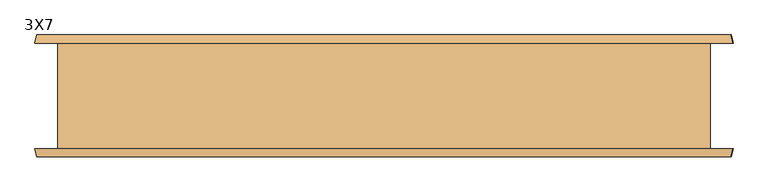
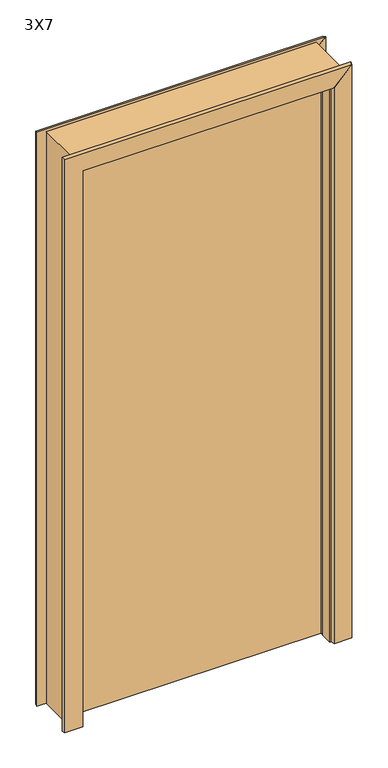
"""IFC4 building model written with IfcOpenShell, lengths in millimetres: door geometry, ASSA ABLOY BE_Doorset_Double Action Door_HardwareSet Info : 3X7."""

from ifc_helpers import new_model, si_unit, point, frame, frame_2d, origin, place, context, project, spatial, polyline, circle_curve, ellipse_curve, trimmed, segment, composite_curve, outline, extrude, faceted_brep, source, transform, mapped, element, save
from ifc_brep_helpers import plane_surface, revolved_surface, advanced_brep


def door_3x7_5d484fb7(model_context):
    return source(origin(), model_context, "Body", "SolidModel", [
        extrude(outline(composite_curve([segment(trimmed(circle_curve(frame_2d((376.3004472, 0.0)), 60.0), [point((430.8440078, 25.0))], [point((430.8440078, -25.0))], False, "CARTESIAN"), True, "CONTINUOUS"), segment(polyline([(430.8440078, -25.0), (-429.2, -25.0), (-429.2, 25.0), (430.8440078, 25.0)]), True, "CONTINUOUS")], self_intersect=False)), frame((0.0, 0.0, 4.0), z_axis=(0.0, 0.0, 1.0), x_axis=(1.0, 0.0, 0.0)), (0.0, 0.0, 1.0), 2096.0),
        advanced_brep(
        [(432.1999993, 29.0558097, 0.0), (432.1999993, 76.2, 0.0), (437.2, 76.2, 0.0), (440.2, 88.2, 0.0), (502.2, 88.2, 0.0), (505.2, 76.2, 0.0), (457.2, 76.2, 0.0), (457.2, -76.2, 0.0), (505.2, -76.2, 0.0), (502.2, -88.2, 0.0), (440.2, -88.2, 0.0), (437.2, -76.2, 0.0), (432.2, -76.2, 0.0), (432.2, -29.0558084, 0.0), (432.1999993, 29.0558097, 2049.9999993), (432.1999993, 76.2, 2049.9999993), (437.2, 76.2, 2055.0), (440.2, 88.2, 2058.0), (502.2, 88.2, 2120.0), (505.2, 76.2, 2123.0), (457.2, 76.2, 2075.0), (457.2, -76.2, 2075.0), (505.2, -76.2, 2123.0), (502.2, -88.2, 2120.0), (440.2, -88.2, 2058.0), (437.2, -76.2, 2055.0), (432.2, -76.2, 2050.0), (432.2, -29.0558084, 2050.0)],
        [
            (0, 1),
            (1, 2),
            (2, 3),
            (3, 4),
            (4, 5),
            (5, 6),
            (6, 7),
            (7, 8),
            (8, 9),
            (9, 10),
            (10, 11),
            (11, 12),
            (12, 13),
            (13, 0, circle_curve(frame((376.3004472, 0.0, 0.0), z_axis=(0.0, 0.0, 1.0), x_axis=(-1.0, 0.0, 0.0)), 63.0)),
            (0, 14),
            (14, 15),
            (15, 1),
            (15, 16),
            (16, 2),
            (16, 17),
            (17, 3),
            (17, 18),
            (18, 4),
            (18, 19),
            (19, 5),
            (19, 20),
            (20, 6),
            (20, 21),
            (21, 7),
            (21, 22),
            (22, 8),
            (22, 23),
            (23, 9),
            (23, 24),
            (24, 10),
            (24, 25),
            (25, 11),
            (25, 26),
            (26, 12),
            (26, 27),
            (27, 13),
            (27, 14, ellipse_curve(frame((376.3004472, 0.0, 1994.1004472), z_axis=(-0.7071067811865507, 0.0, 0.7071067811865445), x_axis=(0.7071067811865445, 0.0, 0.7071067811865505)), 89.0954544, 63.0)),
        ],
        [
            plane_surface(frame((457.2, 76.2, 0.0), z_axis=(0.0, 0.0, -1.0), x_axis=(0.0, -1.0, 0.0))),
            plane_surface(frame((432.1999993, 29.0558097, 0.0), z_axis=(-1.0, 0.0, 0.0), x_axis=(0.0, 0.0, 1.0))),
            plane_surface(frame((432.1999993, 76.2, 0.0), z_axis=(0.0, 1.0, 0.0), x_axis=(0.0, 0.0, 1.0))),
            plane_surface(frame((437.2, 76.2, 0.0), z_axis=(-0.9701425001453396, 0.24253562503630208, 0.0), x_axis=(0.0, 0.0, 1.0))),
            plane_surface(frame((440.2, 88.2, 0.0), z_axis=(0.0, 1.0, 0.0), x_axis=(0.0, 0.0, 1.0))),
            plane_surface(frame((502.2, 88.2, 0.0), z_axis=(0.9701425001453319, 0.24253562503633297, 0.0), x_axis=(0.0, 0.0, 1.0))),
            plane_surface(frame((505.2, 76.2, 0.0), z_axis=(0.0, -1.0, 0.0), x_axis=(0.0, 0.0, 1.0))),
            plane_surface(frame((457.2, 76.2, 0.0), z_axis=(1.0, 0.0, 0.0), x_axis=(0.0, 0.0, 1.0))),
            plane_surface(frame((457.2, -76.2, 0.0), z_axis=(0.0, 1.0, 0.0), x_axis=(0.0, 0.0, 1.0))),
            plane_surface(frame((505.2, -76.2, 0.0), z_axis=(0.9701425001453553, -0.24253562503623965, 0.0), x_axis=(0.0, 0.0, 1.0))),
            plane_surface(frame((502.2, -88.2, 0.0), z_axis=(0.0, -1.0, 0.0), x_axis=(0.0, 0.0, 1.0))),
            plane_surface(frame((440.2, -88.2, 0.0), z_axis=(-0.970142500145363, -0.24253562503620874, 0.0), x_axis=(0.0, 0.0, 1.0))),
            plane_surface(frame((437.2, -76.2, 0.0), z_axis=(0.0, -1.0, 0.0), x_axis=(0.0, 0.0, 1.0))),
            plane_surface(frame((432.2, -76.2, 0.0), z_axis=(-1.0, 0.0, 0.0), x_axis=(0.0, 0.0, 1.0))),
            revolved_surface(polyline([(313.3004472, 0.0, 2057.100447179137), (313.3004472, 0.0, 0.0)]), (376.3004472, 0.0, 0.0), (0.0, 0.0, 1.0)),
            plane_surface(frame((345.6190436, -88.2, 1963.4190436), z_axis=(-0.7071067811865507, 0.0, 0.7071067811865445), x_axis=(0.0, 1.0, 0.0))),
        ],
        [
            (0, [[1, 2, 3, 4, 5, 6, 7, 8, 9, 10, 11, 12, 13, 14]]),
            (1, [[-1, 15, 16, 17]]),
            (2, [[-2, -17, 18, 19]]),
            (3, [[-3, -19, 20, 21]]),
            (4, [[-4, -21, 22, 23]]),
            (5, [[-5, -23, 24, 25]]),
            (6, [[-6, -25, 26, 27]]),
            (7, [[-7, -27, 28, 29]]),
            (8, [[-8, -29, 30, 31]]),
            (9, [[-9, -31, 32, 33]]),
            (10, [[-10, -33, 34, 35]]),
            (11, [[-11, -35, 36, 37]]),
            (12, [[-12, -37, 38, 39]]),
            (13, [[-13, -39, 40, 41]]),
            (14, [[-14, -41, 42, -15]]),
            (15, [[-16, -42, -40, -38, -36, -34, -32, -30, -28, -26, -24, -22, -20, -18]]),
        ],
    ),
        faceted_brep([(-432.1999993, -76.2, 0.0), (-437.2, -76.2, 0.0), (-440.2, -88.2, 0.0), (-502.2, -88.2, 0.0), (-505.2, -76.2, 0.0), (-457.2, -76.2, 0.0), (-457.2, 76.2, 0.0), (-505.2, 76.2, 0.0), (-502.2, 88.2, 0.0), (-440.2, 88.2, 0.0), (-437.2, 76.2, 0.0), (-432.1999993, 76.2, 0.0), (-432.1999993, -76.2, 2049.9999993), (432.1999993, -76.2, 2049.9999993), (437.2, -76.2, 2055.0), (-437.2, -76.2, 2055.0), (-440.2, -88.2, 2058.0), (440.2, -88.2, 2058.0), (502.2, -88.2, 2120.0), (-502.2, -88.2, 2120.0), (-505.2, -76.2, 2123.0), (505.2, -76.2, 2123.0), (457.2, -76.2, 2075.0), (-457.2, -76.2, 2075.0), (-457.2, 76.2, 2075.0), (457.2, 76.2, 2075.0), (505.2, 76.2, 2123.0), (-505.2, 76.2, 2123.0), (-502.2, 88.2, 2120.0), (502.2, 88.2, 2120.0), (440.2, 88.2, 2058.0), (-440.2, 88.2, 2058.0), (-437.2, 76.2, 2055.0), (437.2, 76.2, 2055.0), (432.1999993, 76.2, 2049.9999993), (-432.1999993, 76.2, 2049.9999993)], [[[0, 1, 2, 3, 4, 5, 6, 7, 8, 9, 10, 11]], [[1, 0, 12, 13, 14, 15]], [[2, 1, 15, 16]], [[3, 2, 16, 17, 18, 19]], [[4, 3, 19, 20]], [[5, 4, 20, 21, 22, 23]], [[6, 5, 23, 24]], [[7, 6, 24, 25, 26, 27]], [[8, 7, 27, 28]], [[9, 8, 28, 29, 30, 31]], [[10, 9, 31, 32]], [[11, 10, 32, 33, 34, 35]], [[0, 11, 35, 12]], [[12, 35, 34, 13]], [[32, 31, 30, 33]], [[28, 27, 26, 29]], [[24, 23, 22, 25]], [[21, 20, 19, 18]], [[16, 15, 14, 17]], [[13, 34, 33, 30, 29, 26, 25, 22, 21, 18, 17, 14]]]),
        extrude(outline(polyline([(0.0, -472.2), (0.0, -457.2), (2100.0, -457.2), (2100.0, 457.2), (0.0, 457.2), (0.0, 472.2), (2115.0, 472.2), (2115.0, -472.2), (0.0, -472.2)])), frame((0.0, -76.2, 0.0), z_axis=(0.0, 1.0, 0.0), x_axis=(0.0, 0.0, 1.0)), (0.0, 0.0, 1.0), 152.4),
    ])


if __name__ == "__main__":
    model = new_model("IFC4")
    model_context = context("Model", 3, world=origin())
    ifc_project = project(units=[si_unit("LENGTHUNIT", "METRE", prefix="MILLI")], contexts=[model_context])
    site = spatial("IfcSite", under=ifc_project)
    building = spatial("IfcBuilding", under=site)
    placement = place(None, origin())
    door_3x7_shape = door_3x7_5d484fb7(model_context)
    element("IfcDoor", 1, ObjectType="ASSA ABLOY BE_Doorset_Double Action Door_HardwareSet Info : 3X7", at=placement, inside=building, context=model_context, shape_type="MappedRepresentation", body=[
        mapped(door_3x7_shape, transform((0.0, 0.0, 0.0), x_axis=(1.0, 0.0, 0.0), y_axis=(0.0, 1.0, 0.0), z_axis=(0.0, 0.0, 1.0))),
    ])
    save(model, "model.ifc")

# Revit data of these elements
# Type "ASSA ABLOY BE_Doorset_Double Action Door_HardwareSet Info : 3X7"
#   Type Mark = "45"
#   Uniclass 2.0 Description = "Doorsets"
#   Uniclass 2.0 Code = "PR-59-23"
#   Uniclass 1.4 Description = "Doors"
#   Uniclass 1.4 Code = "JL20"
#   URL = "http://www.assaabloy.be/door-solutions/double-action-door-solution"
#   UNSPSC Code = "301715"
#   Type Comments = "1380x2110 (1430X2135)"
#   Region Europe = "BE, LU"
#   Provider = "ASSA ABLOY Belgium"
#   Product Guid = "1d6185b8-f4a7-4cd1-8e4c-530cf6da835d"
#   OmniClass Description = "Doors"
#   OmniClass Code = "23-17 11 00"
#   Name = "Double Action Door Solution"
#   NBS Reference Description = "Doorsets"
#   NBS Reference Code = "59-23"
#   Model = "ASSA ABLOY BE_Doorset_Double Action Door_HardwareSet Info"
#   Manufacturer = "ASSA ABLOY"
#   Lock Cases = "A56D5_D5_by Litto ASSA ABLOY"
#   IFC Classification = "Door"
#   Hardware Set = "A-S-1-DC475-BE04"
#   Door Closers = "DC475_Cam-Motion®_by ASSA ABLOY"
#   Description = "The ASSA ABLOY Belgium solution for Interior double action self-closing door equipped with a Cam-Motion® Floor Spring for an easier opening. This solution can also be used for two-way movement fire rated doors."
#   Date of publishing = "2016-03-04"
#   Contact Provider = "http://www.assaabloy.be/contact-solutions-team"
#   BIMobject category = "Door Sets"
#   BIMobject Unique ref = "A-S-1-DC475-BE04"
#   BIMobject Product Page = "http://bimobject.com/en/assaabloy-be/product/A-S-1-DC475-BE04"
#   BIMobject Product Group = "Single-Wood-Self Closing"
#   BIMobject Product Family = "Interior Door Solutions"
#   BIMobject Instructions Video = "https://www.youtube.com/watch?v=sh1CO-2jNM0"
#   BIMobject Brand = "ASSA ABLOY BE"
#   Architectural and Accessory Hardware = "TL0452SS_TONIC LINE_by Litto ASSA ABLOY"
#   Analytic Construction = "<None>"
#   Min Door Width = 2' - 0.80315"
#   Min Door Height = 6' - 11.07087"
#   Max Door Width = 4' - 6.33071"
#   Max Door Height = 6' - 10.67717"
#   Thickness = 0' - 1.9685"
#   Rough Width = 3' - 1.1811"
#   Rough Height = 6' - 11.26772"
#   Height = 6' - 10.67717"
#   Width = 3' - 0"
#   Frame Depth [instance default] = 0' - 9.84252"
#   Door Panel Width = 2' - 10.4252"
#   Frame Width = 3' - 0"
#   Frame Height = 7' - 0"
#   Edition number = 1
#   Frame Material = Wood
#   Frame Finish = Light Grey
#   Door Material = Wood
#   Door Finish = Light Grey
#   Function = (empty or 0)
#   Wall Closure = (empty or 0)
# Element 1 (IfcDoor, "ASSA ABLOY BE_Doorset_Double Action Door_HardwareSet Info : 3X7")
#   Frame Depth = 0' - 6"
#   Materials on its faces: "Light Grey"
# Materials
#   "Wood": class "Generic", colour RGB 170 151 133, transparency 0, Cost = 0
#   "Light Grey": class "Unassigned", colour RGB 200 200 200, transparency 0, Cost = 0
